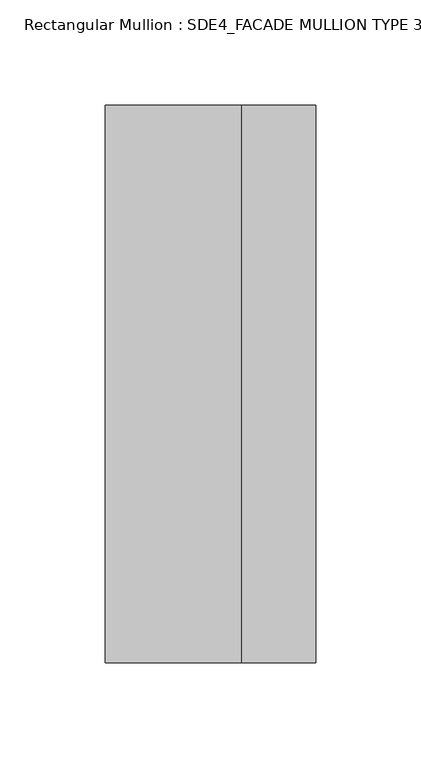
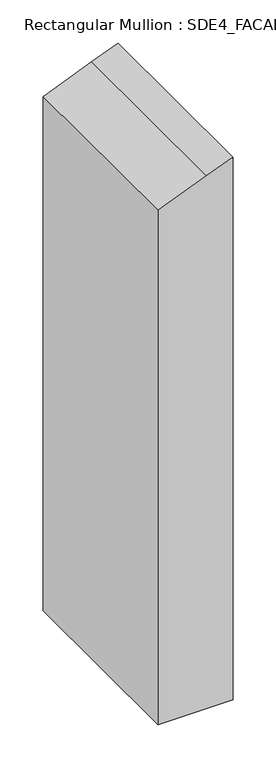
"""IFC4 building model written with IfcOpenShell, lengths in millimetres: member geometry, Rectangular Mullion : SDE4_FACADE MULLION TYPE 3."""

from ifc_helpers import new_model, si_unit, frame, origin, place, context, project, spatial, polyline, outline, extrude, source, transform, mapped, element, save


def rectangular_mullion_sde4_facade_mullion_type_3_9a51d8d2(model_context):
    return source(origin(), model_context, "Body", "SweptSolid", [
        extrude(outline(polyline([(-23.0813185, 50.0), (-37.1390676, 14.8556271), (-63.0813185, -50.0), (-787.974544, -50.0), (-787.974544, 50.0), (-23.0813185, 50.0)])), frame((0.0, -132.5, 0.0), z_axis=(0.0, 1.0, 0.0), x_axis=(0.0, 0.0, 1.0)), (0.0, 0.0, 1.0), 265.0),
    ])


if __name__ == "__main__":
    model = new_model("IFC4")
    model_context = context("Model", 3, world=origin())
    ifc_project = project(units=[si_unit("LENGTHUNIT", "METRE", prefix="MILLI")], contexts=[model_context])
    site = spatial("IfcSite", under=ifc_project)
    building = spatial("IfcBuilding", under=site)
    placement = place(None, origin())
    rectangular_mullion_sde4_facade_mullion_type_3_shape = rectangular_mullion_sde4_facade_mullion_type_3_9a51d8d2(model_context)
    element("IfcMember", 1, ObjectType="Rectangular Mullion : SDE4_FACADE MULLION TYPE 3", at=placement, inside=building, context=model_context, shape_type="MappedRepresentation", body=[
        mapped(rectangular_mullion_sde4_facade_mullion_type_3_shape, transform((0.0, 0.0, 0.0), x_axis=(1.0, 0.0, 0.0), y_axis=(0.0, 1.0, 0.0), z_axis=(0.0, 0.0, 1.0))),
    ])
    save(model, "model.ifc")

# Revit data of these elements
# Type "Rectangular Mullion : SDE4_FACADE MULLION TYPE 3"
#   built-in parameter 1007322 = 0.869423 (stored number, unit not read)
#   built-in parameter 1007321 = 0.164042 (stored number, unit not read)
#   built-in parameter 1007320 = 0.164042 (stored number, unit not read)
